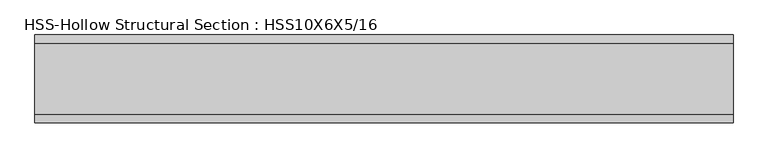
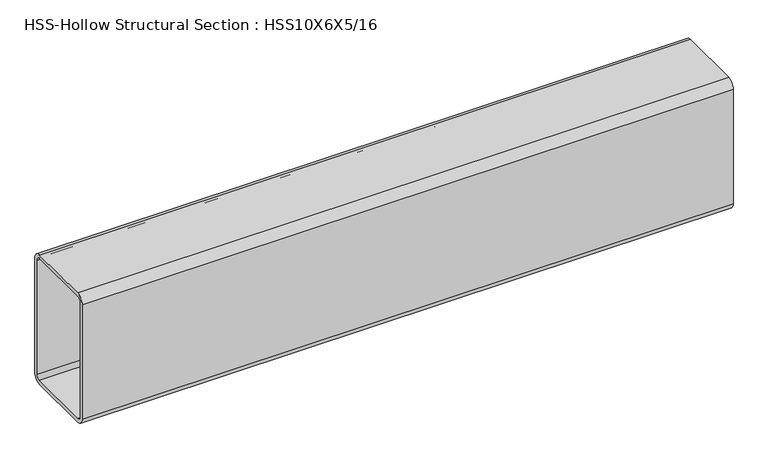
"""IFC4 building model written with IfcOpenShell, lengths in millimetres: beam geometry, HSS-Hollow Structural Section : HSS10X6X5/16."""

from ifc_helpers import new_model, si_unit, point, frame, frame_2d, origin, place, context, project, spatial, polyline, circle_curve, trimmed, segment, composite_curve, outline, extrude, source, transform, mapped, element, save


def hss_hollow_structural_section_hss10x6x5_16_419a5111(model_context):
    return source(origin(), model_context, "Body", "SweptSolid", [
        extrude(outline(composite_curve([segment(polyline([(76.2, 112.2172), (76.2, -112.2172)]), True, "CONTINUOUS"), segment(trimmed(circle_curve(frame_2d((61.4172, -112.2172)), 14.7828), [point((76.2, -112.2172))], [point((61.4172, -127.0))], False, "CARTESIAN"), True, "CONTINUOUS"), segment(polyline([(61.4172, -127.0), (-61.4172, -127.0)]), True, "CONTINUOUS"), segment(trimmed(circle_curve(frame_2d((-61.4172, -112.2172)), 14.7828), [point((-61.4172, -127.0))], [point((-76.2, -112.2172))], False, "CARTESIAN"), True, "CONTINUOUS"), segment(polyline([(-76.2, -112.2172), (-76.2, 112.2172)]), True, "CONTINUOUS"), segment(trimmed(circle_curve(frame_2d((-61.4172, 112.2172)), 14.7828), [point((-76.2, 112.2172))], [point((-61.4172, 127.0))], False, "CARTESIAN"), True, "CONTINUOUS"), segment(polyline([(-61.4172, 127.0), (61.4172, 127.0)]), True, "CONTINUOUS"), segment(trimmed(circle_curve(frame_2d((61.4172, 112.2172)), 14.7828), [point((61.4172, 127.0))], [point((76.2, 112.2172))], False, "CARTESIAN"), True, "CONTINUOUS")], self_intersect=False), holes=[composite_curve([segment(trimmed(circle_curve(frame_2d((-61.4172, 112.2172)), 7.3914), [point((-61.4172, 119.6086))], [point((-68.8086, 112.2172))], True, "CARTESIAN"), True, "CONTINUOUS"), segment(polyline([(-68.8086, 112.2172), (-68.8086, -112.2172)]), True, "CONTINUOUS"), segment(trimmed(circle_curve(frame_2d((-61.4172, -112.2172)), 7.3914), [point((-68.8086, -112.2172))], [point((-61.4172, -119.6086))], True, "CARTESIAN"), True, "CONTINUOUS"), segment(polyline([(-61.4172, -119.6086), (61.4172, -119.6086)]), True, "CONTINUOUS"), segment(trimmed(circle_curve(frame_2d((61.4172, -112.2172)), 7.3914), [point((61.4172, -119.6086))], [point((68.8086, -112.2172))], True, "CARTESIAN"), True, "CONTINUOUS"), segment(polyline([(68.8086, -112.2172), (68.8086, 112.2172)]), True, "CONTINUOUS"), segment(trimmed(circle_curve(frame_2d((61.4172, 112.2172)), 7.3914), [point((68.8086, 112.2172))], [point((61.4172, 119.6086))], True, "CARTESIAN"), True, "CONTINUOUS"), segment(polyline([(61.4172, 119.6086), (-61.4172, 119.6086)]), True, "CONTINUOUS")], self_intersect=False)]), frame((-605.0327521, 0.0, 0.0), z_axis=(1.0, 0.0, 0.0), x_axis=(0.0, 1.0, 0.0)), (0.0, 0.0, 1.0), 1210.0655043),
    ])


if __name__ == "__main__":
    model = new_model("IFC4")
    model_context = context("Model", 3, world=origin())
    ifc_project = project(units=[si_unit("LENGTHUNIT", "METRE", prefix="MILLI")], contexts=[model_context])
    site = spatial("IfcSite", under=ifc_project)
    building = spatial("IfcBuilding", under=site)
    placement = place(None, origin())
    hss_hollow_structural_section_hss10x6x5_16_shape = hss_hollow_structural_section_hss10x6x5_16_419a5111(model_context)
    element("IfcBeam", 1, ObjectType="HSS-Hollow Structural Section : HSS10X6X5/16", at=placement, inside=building, context=model_context, shape_type="MappedRepresentation", body=[
        mapped(hss_hollow_structural_section_hss10x6x5_16_shape, transform((0.0, 0.0, 0.0), x_axis=(1.0, 0.0, 0.0), y_axis=(0.0, 1.0, 0.0), z_axis=(0.0, 0.0, 1.0))),
    ])
    save(model, "model.ifc")

# Revit data of these elements
# Type "HSS-Hollow Structural Section : HSS10X6X5/16"
#   Assembly Code = "B10"
#   Shape = "Rect."
#   W = 31.8
#   Ht = 0' - 10"
#   Length [instance default] = 5' - 0"
#   b = 0' - 6"
#   kr = 0' - 0.582"
#   t = 0' - 0.291"
#   A = 0.0608333 SF
#   Structural Material [instance default] = Steel ASTM A500, Grade B, Rectangular and Square
# Element 1 (IfcBeam, "HSS-Hollow Structural Section : HSS10X6X5/16")
#   Structural Material = Steel ASTM A992
#   Materials on its faces: "Steel ASTM A992"
# Materials
#   "Steel ASTM A500, Grade B, Rectangular and Square": class "Metal", colour RGB 199 199 199, transparency 0, Description = "Carbon steel", Cost = 0
#   "Steel ASTM A992": class "Metal", colour RGB 199 199 199, transparency 0, Description = "Structural steel 50ksi", Cost = 0
